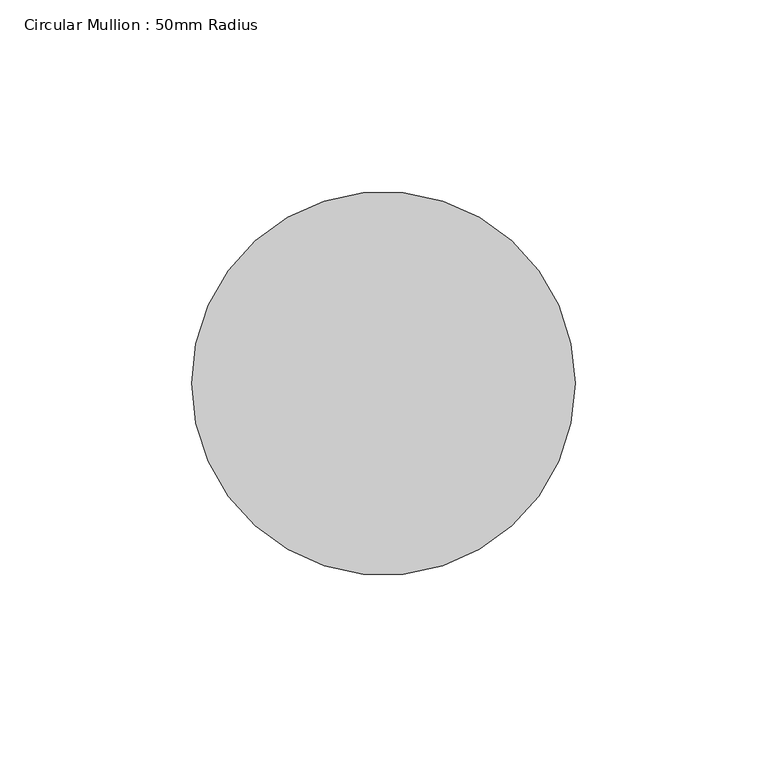
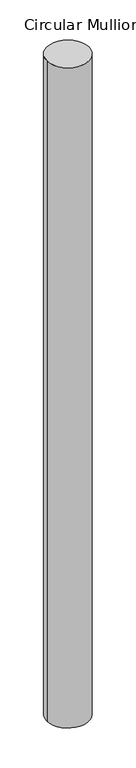
"""IFC4 building model written with IfcOpenShell, lengths in millimetres: member geometry, Circular Mullion : 50mm Radius."""

from ifc_helpers import new_model, si_unit, point, frame, origin, origin_2d, place, context, project, spatial, circle_curve, trimmed, segment, composite_curve, outline, extrude, source, transform, mapped, element, save


def circular_mullion_50mm_radius_706dd157(model_context):
    return source(origin(), model_context, "Body", "SweptSolid", [
        extrude(outline(composite_curve([segment(trimmed(circle_curve(origin_2d(), 50.0), [point((50.0, 0.0))], [point((-50.0, 0.0))], False, "CARTESIAN"), True, "CONTINUOUS"), segment(trimmed(circle_curve(origin_2d(), 50.0), [point((-50.0, 0.0))], [point((50.0, 0.0))], False, "CARTESIAN"), True, "CONTINUOUS")], self_intersect=False)), frame((0.0, 0.0, -1660.4007158), z_axis=(0.0, 0.0, 1.0), x_axis=(1.0, 0.0, 0.0)), (0.0, 0.0, 1.0), 1660.4007158),
    ])


if __name__ == "__main__":
    model = new_model("IFC4")
    model_context = context("Model", 3, world=origin())
    ifc_project = project(units=[si_unit("LENGTHUNIT", "METRE", prefix="MILLI")], contexts=[model_context])
    site = spatial("IfcSite", under=ifc_project)
    building = spatial("IfcBuilding", under=site)
    placement = place(None, origin())
    circular_mullion_50mm_radius_shape = circular_mullion_50mm_radius_706dd157(model_context)
    element("IfcMember", 1, ObjectType="Circular Mullion : 50mm Radius", at=placement, inside=building, context=model_context, shape_type="MappedRepresentation", body=[
        mapped(circular_mullion_50mm_radius_shape, transform((0.0, 0.0, 0.0), x_axis=(1.0, 0.0, 0.0), y_axis=(0.0, 1.0, 0.0), z_axis=(0.0, 0.0, 1.0))),
    ])
    save(model, "model.ifc")

# Revit data of these elements
# Type "Circular Mullion : 50mm Radius"
#   built-in parameter 1007350 = 0.164042 (stored number, unit not read)
# Element 1 (IfcMember, "Circular Mullion : 50mm Radius")
#   Materials on its faces: "Aluminium"
# Materials
#   "Aluminium": class "Metal", colour RGB 247 247 247, transparency 0, Description = "Aluminium 6061", Cost = 0
